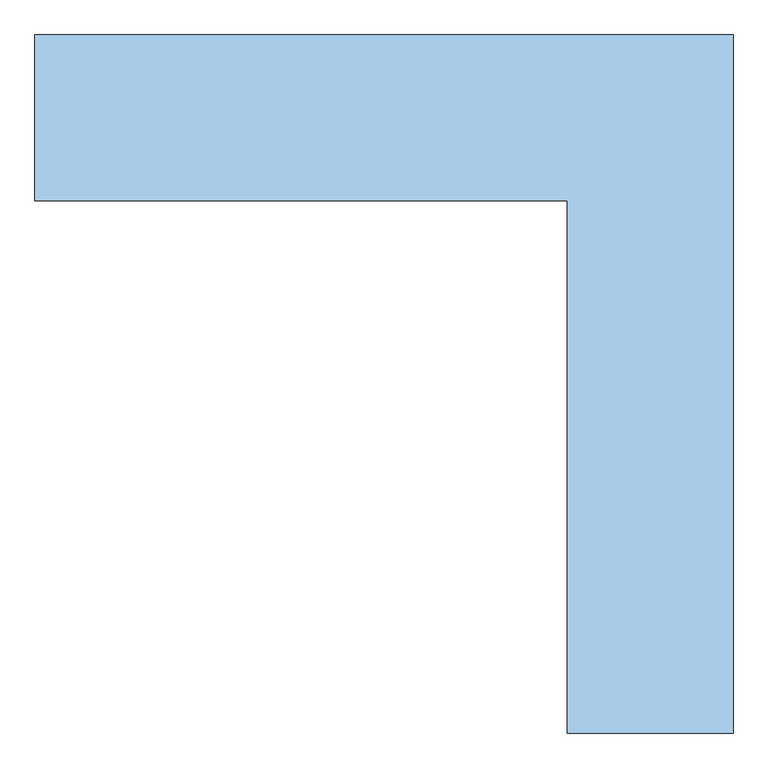
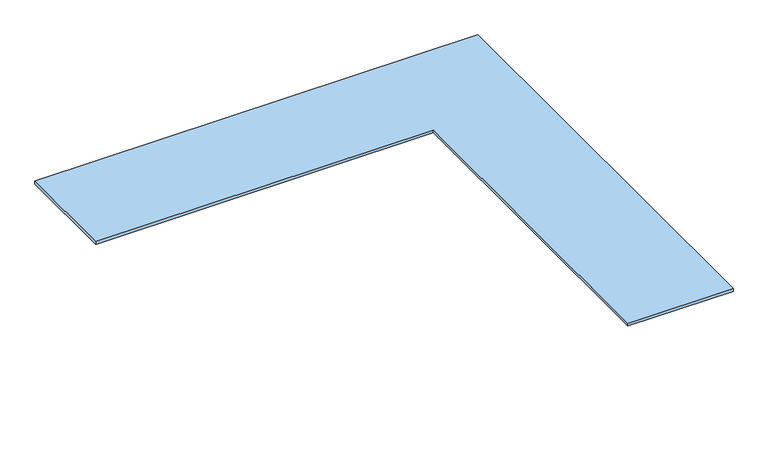
"""IFC4 building model written with IfcOpenShell, lengths in millimetres: window geometry, .CC_ND 300_PEDRA PEITORIL EM L : 3.06F x 3.06E x 0.73L."""

from ifc_helpers import new_model, si_unit, frame, origin, place, context, project, spatial, polyline, outline, extrude, source, transform, mapped, element, save


def window_829f86a1(model_context):
    return source(origin(), model_context, "Body", "SweptSolid", [
        extrude(outline(polyline([(-1265.0, -98.8), (-1265.0, 628.8), (1795.0, 628.8), (1795.0, -2431.2), (1067.4, -2431.2), (1067.4, -98.8), (-1265.0, -98.8)])), frame((0.0, 0.0, 900.0), z_axis=(0.0, 0.0, 1.0), x_axis=(1.0, 0.0, 0.0)), (0.0, 0.0, 1.0), 20.0),
    ])


if __name__ == "__main__":
    model = new_model("IFC4")
    model_context = context("Model", 3, world=origin())
    ifc_project = project(units=[si_unit("LENGTHUNIT", "METRE", prefix="MILLI")], contexts=[model_context])
    site = spatial("IfcSite", under=ifc_project)
    building = spatial("IfcBuilding", under=site)
    placement = place(None, origin())
    window_shape = window_829f86a1(model_context)
    element("IfcWindow", 1, ObjectType=".CC_ND 300_PEDRA PEITORIL EM L : 3.06F x 3.06E x 0.73L", at=placement, inside=building, context=model_context, shape_type="MappedRepresentation", body=[
        mapped(window_shape, transform((0.0, 0.0, 0.0), x_axis=(1.0, 0.0, 0.0), y_axis=(0.0, 1.0, 0.0), z_axis=(0.0, 0.0, 1.0))),
    ])
    save(model, "model.ifc")

# Revit data of these elements
# Type ".CC_ND 300_PEDRA PEITORIL EM L : 3.06F x 3.06E x 0.73L"
#   Type Mark = "63"
#   Largura da pedra da frente [instance default] = 0.26 m
#   Largura da pedra da esquerda [instance default] = 0.26 m
#   Extensão esquerda interna [instance default] = 0.03 m
#   Extensão esquerda externa [instance default] = 0.03 m
#   Comprimento Esquerda = 2.3324 m
#   Extensão frente interna [instance default] = 0.03 m
#   Extensão frente externa [instance default] = 0.03 m
#   Espessura peitoril = 0.02 m
#   Espessura da parede [instance default] = 0.20 m
#   Comprimento da pedra [instance default] = 4.8624 m
#   Comprimento Frente = 2.53 m
#   Altura-padrão do peitoril [instance default] = 0.90 m
#   Pedra do peitoril = .GRANITO_BRANCO_ITAUNAS
#   Rough Width = 0
#   Rough Height = 0
#   Height = 0
#   Wall Closure = (empty or 0)
#   Width = 0
# Element 1 (IfcWindow, ".CC_ND 300_PEDRA PEITORIL EM L : 3.06F x 3.06E x 0.73L")
#   Largura da pedra da frente = 0.7276 m
#   Largura da pedra da esquerda = 0.7276 m
#   Extensão esquerda interna = 0.00 m
#   Extensão esquerda externa = 0.53 m
#   Extensão frente interna = 0.00 m
#   Extensão frente externa = 0.53 m
#   Espessura da parede = 0.1976 m
#   Materials on its faces: ".GRANITO_BRANCO_ITAUNAS"
# Materials
#   ".GRANITO_BRANCO_ITAUNAS": class ".CC_PEDRA REVEST.", colour RGB 202 195 174, transparency 0, Description = "Revestimento em granito", Cost = 0
